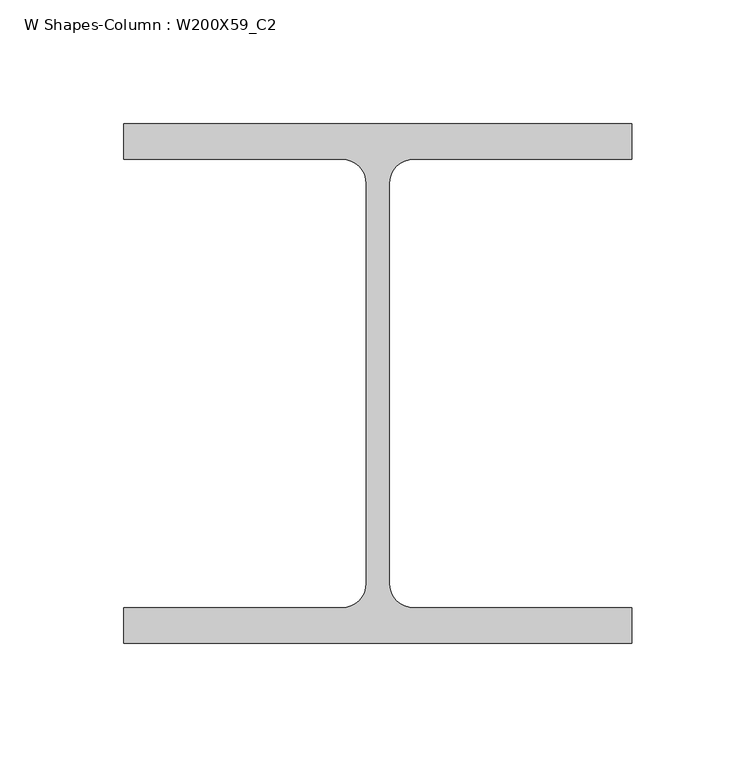
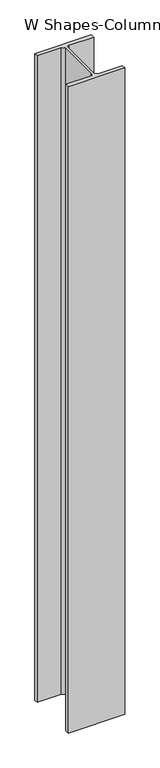
"""IFC4 building model written with IfcOpenShell, lengths in millimetres: column geometry, W Shapes-Column : W200X59_C2."""

from ifc_helpers import new_model, si_unit, point, frame, frame_2d, origin, place, context, project, spatial, polyline, circle_curve, trimmed, segment, composite_curve, outline, extrude, source, transform, mapped, element, save


def w_shapes_column_w200x59_c2_281d749c(model_context):
    return source(origin(), model_context, "Body", "SweptSolid", [
        extrude(outline(composite_curve([segment(polyline([(102.489, 104.775), (102.489, 90.551), (14.5796, 90.551)]), True, "CONTINUOUS"), segment(trimmed(circle_curve(frame_2d((14.5796, 80.5434)), 10.0076), [point((14.5796, 90.551))], [point((4.572, 80.5434))], True, "CARTESIAN"), True, "CONTINUOUS"), segment(polyline([(4.572, 80.5434), (4.572, -80.5434)]), True, "CONTINUOUS"), segment(trimmed(circle_curve(frame_2d((14.5796, -80.5434)), 10.0076), [point((4.572, -80.5434))], [point((14.5796, -90.551))], True, "CARTESIAN"), True, "CONTINUOUS"), segment(polyline([(14.5796, -90.551), (102.489, -90.551), (102.489, -104.775), (-102.489, -104.775), (-102.489, -90.551), (-14.5796, -90.551)]), True, "CONTINUOUS"), segment(trimmed(circle_curve(frame_2d((-14.5796, -80.5434)), 10.0076), [point((-14.5796, -90.551))], [point((-4.572, -80.5434))], True, "CARTESIAN"), True, "CONTINUOUS"), segment(polyline([(-4.572, -80.5434), (-4.572, 80.5434)]), True, "CONTINUOUS"), segment(trimmed(circle_curve(frame_2d((-14.5796, 80.5434)), 10.0076), [point((-4.572, 80.5434))], [point((-14.5796, 90.551))], True, "CARTESIAN"), True, "CONTINUOUS"), segment(polyline([(-14.5796, 90.551), (-102.489, 90.551), (-102.489, 104.775), (102.489, 104.775)]), True, "CONTINUOUS")], self_intersect=False)), frame((0.0, 0.0, 506.0), z_axis=(0.0, 0.0, 1.0), x_axis=(1.0, 0.0, 0.0)), (0.0, 0.0, 1.0), 2484.0),
    ])


if __name__ == "__main__":
    model = new_model("IFC4")
    model_context = context("Model", 3, world=origin())
    ifc_project = project(units=[si_unit("LENGTHUNIT", "METRE", prefix="MILLI")], contexts=[model_context])
    site = spatial("IfcSite", under=ifc_project)
    building = spatial("IfcBuilding", under=site)
    placement = place(None, origin())
    w_shapes_column_w200x59_c2_shape = w_shapes_column_w200x59_c2_281d749c(model_context)
    element("IfcColumn", 1, ObjectType="W Shapes-Column : W200X59_C2", at=placement, inside=building, context=model_context, shape_type="MappedRepresentation", body=[
        mapped(w_shapes_column_w200x59_c2_shape, transform((0.0, 0.0, 0.0), x_axis=(1.0, 0.0, 0.0), y_axis=(0.0, 1.0, 0.0), z_axis=(0.0, 0.0, 1.0))),
    ])
    save(model, "model.ifc")

# Revit data of these elements
# Type "W Shapes-Column : W200X59_C2"
#   Section Name Key = "W8x40"
#   Assembly Code = "B10"
#   Width = 20.4978 cm
#   Web Thickness = 0.9144 cm
#   Web Fillet = 1.0008 cm
#   Warping Constant = 194957.0 cm⁶
#   Torsional Moment of Inertia = 46.6179 cm⁴
#   Section Area = 75.4837 cm²
#   Plastic Modulus weak axis = 303.161 cm³
#   Plastic Modulus strong axis = 652.205 cm³
#   Perimeter = 1.20396 m²/m
#   Nominal Weight = 59.5266 kgf/m
#   Moment of Inertia weak axis = 2043.70 cm⁴
#   Moment of Inertia strong axis = 6076.98 cm⁴
#   Height = 20.955 cm
#   Flange Thickness = 1.4224 cm
#   Elastic Modulus weak axis = 199.922 cm³
#   Elastic Modulus strong axis = 581.741 cm³
#   Clear Web Height = 19.05 cm
#   Centroid Vertical = 10.4775 cm
#   Centroid Horizontal = 10.2489 cm
#   Bolt Spacing = 13.97 cm
#   Structural Material [instance default] = Steel ASTM A992
#   Principal Axes Angle = 0
# Element 1 (IfcColumn, "W Shapes-Column : W200X59_C2")
#   Structural Material = none
# Materials
#   "Steel ASTM A992": class "Metal", colour RGB 199 199 199, transparency 0, Description = "Structural steel 50ksi", Cost = 0
